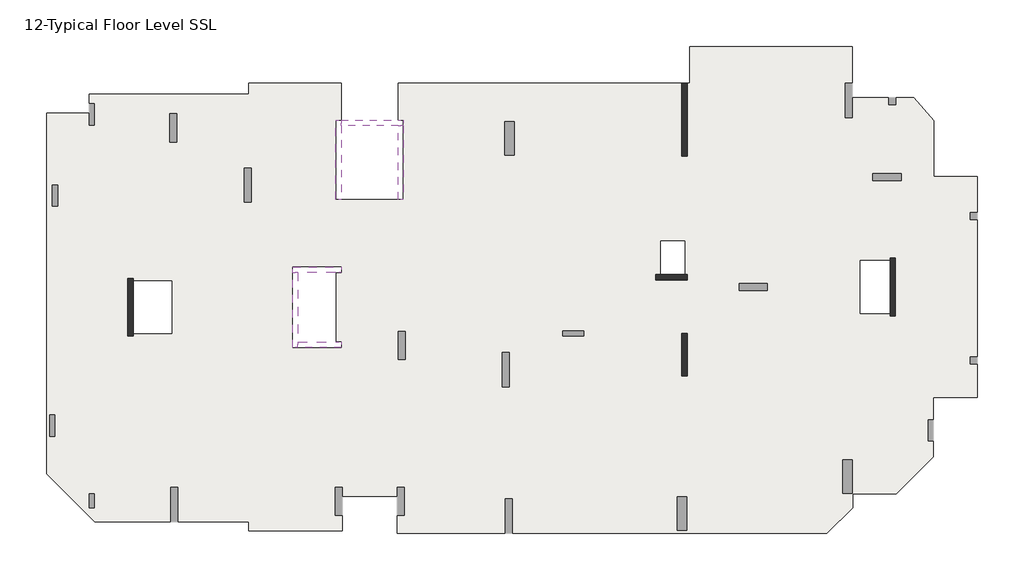
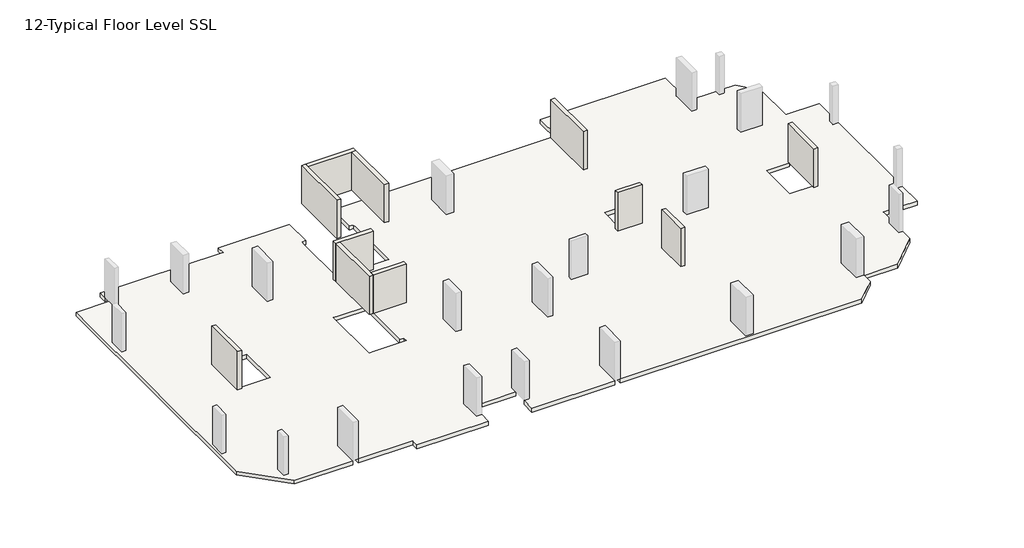
# One storey, part 1 of 2: 11 walls, 1 slab.
"""IFC4 building model written with IfcOpenShell, lengths in millimetres."""

from ifc_helpers import new_model, si_unit, origin, place, context, project, spatial, faceted_brep, element, save

model = new_model("IFC4")

# Units and contexts
model_context = context("Model", 3, world=origin())
ifc_project = project(units=[si_unit("LENGTHUNIT", "METRE", prefix="MILLI")], contexts=[model_context])

# Site, building, storey
site = spatial("IfcSite", under=ifc_project)
building = spatial("IfcBuilding", under=site)
storey = spatial("IfcBuildingStorey", under=building, Name="12-Typical Floor Level SSL", Elevation=30000.0)

# Slab
placement = place(None, origin())
element("IfcSlab", 1, ObjectType="Generic 300mm", at=placement, inside=storey, context=model_context, shape_type="Brep", body=[
    faceted_brep([(36192.0021644, 24072.000519, 29700.0), (36192.0021644, 26172.000519, 29700.0), (45446.0007483, 26172.000519, 29700.0), (45446.0007483, 24087.0, 29700.0), (45046.0007483, 24087.0, 29700.0), (45046.0007483, 22137.0, 29700.0), (45446.0007483, 22137.0, 29700.0), (45446.0007483, 23252.0000315, 29700.0), (47498.6337868, 23252.0000315, 29700.0), (47498.6337868, 22852.0, 29700.0), (47898.6337868, 22852.0, 29700.0), (47898.6337868, 23252.0000315, 29700.0), (48936.764334, 23252.0000315, 29700.0), (50076.0016214, 21956.8283806, 29700.0), (50076.0016214, 18780.0084406, 29700.0), (52549.9999998, 18780.0084406, 29700.0), (52549.9999998, 16712.0, 29700.0), (52149.9999998, 16712.0, 29700.0), (52149.9999998, 16312.0, 29700.0), (52549.9999998, 16312.0, 29700.0), (52549.9999998, 8504.0039609, 29700.0), (52149.9999998, 8504.0039609, 29700.0), (52149.9999998, 8104.0039609, 29700.0), (52549.9999998, 8104.0039609, 29700.0), (52549.9999998, 6204.0084406, 29700.0), (50046.0009271, 6204.0084406, 29700.0), (50046.0009271, 4931.9999929, 29700.0), (49746.0009271, 4931.9999929, 29700.0), (49746.0009271, 3731.9999929, 29700.0), (50046.0009271, 3731.9999929, 29700.0), (50046.0009271, 2810.5958657, 29700.0), (47943.4055804, 708.000519, 29700.0), (45456.0017287, 708.000519, 29700.0), (45456.0017287, -61.7051085, 29700.0), (43990.7023722, -1527.004465, 29700.0), (26113.9999998, -1527.004465, 29700.0), (26113.9999998, 422.995535, 29700.0), (25713.9999998, 422.995535, 29700.0), (25713.9999998, -1527.004465, 29700.0), (19569.9997488, -1527.004465, 29700.0), (19569.9997488, -512.0044652, 29700.0), (19969.9997488, -512.0044652, 29700.0), (19969.9997488, 1087.9955348, 29700.0), (19569.9997488, 1087.9955348, 29700.0), (19569.9997488, 564.000519, 29700.0), (16429.9999981, 564.000519, 29700.0), (16429.9999981, 1088.0, 29700.0), (16029.9999981, 1088.0, 29700.0), (16029.9999981, -512.0, 29700.0), (16429.9999981, -512.0, 29700.0), (16429.9999981, -1391.999481, 29700.0), (11136.0000923, -1391.999481, 29700.0), (11136.0000923, -866.9999847, 29700.0), (7082.0000416, -866.9999847, 29700.0), (7082.0000416, 1083.0000153, 29700.0), (6682.0000416, 1083.0000153, 29700.0), (6682.0000416, -866.9999847, 29700.0), (2364.4419097, -866.9999847, 29700.0), (-372.0, 1869.441925, 29700.0), (-372.0, 22380.0004589, 29700.0), (2052.0, 22380.0004589, 29700.0), (2052.0, 21708.0000656, 29700.0), (2352.0, 21708.0000656, 29700.0), (2352.0, 22908.0000656, 29700.0), (2052.0, 22908.0000656, 29700.0), (2052.0, 23472.000519, 29700.0), (11136.0000923, 23472.000519, 29700.0), (11136.0000923, 24072.000519, 29700.0), (16380.0000168, 24072.000519, 29700.0), (16380.0000168, 21972.0, 29700.0), (16079.9999997, 21972.0, 29700.0), (16079.9999997, 21672.0, 29700.0), (16079.9999997, 17468.0, 29700.0), (16379.9999997, 17468.0, 29700.0), (19619.9999997, 17468.0, 29700.0), (19919.9999997, 17468.0, 29700.0), (19919.9999997, 21672.0, 29700.0), (19919.9999997, 21972.0, 29700.0), (19619.9997365, 21972.0, 29700.0), (19619.9997365, 24072.000519, 29700.0), (35747.9999998, 24072.000519, 29700.0), (35747.9999998, 19932.0, 29700.0), (36047.9999998, 19932.0, 29700.0), (36047.9999998, 24072.000519, 29700.0), (16079.9999907, 9359.999998, 29700.0), (16079.9999907, 13320.0000002, 29700.0), (16380.0000168, 13320.0000002, 29700.0), (16380.0000168, 13620.0000002, 29700.0), (13919.9999907, 13620.0000002, 29700.0), (13619.9999907, 13620.0000002, 29700.0), (13619.9999907, 13320.0000002, 29700.0), (13619.9999907, 9359.999998, 29700.0), (13619.9999907, 9059.999998, 29700.0), (13919.9999907, 9059.999998, 29700.0), (16380.0000168, 9059.999998, 29700.0), (16380.0000168, 9359.999998, 29700.0), (4548.0000034, 9840.0000003, 29700.0), (6743.9999995, 9840.0000003, 29700.0), (6743.9999995, 12840.0000003, 29700.0), (4548.0000034, 12840.0000003, 29700.0), (4548.0000025, 12984.0000001, 29700.0), (4248.0000025, 12984.0000001, 29700.0), (4248.0000025, 9696.0, 29700.0), (4548.0000025, 9696.0, 29700.0), (47580.0014798, 13992.0079177, 29700.0), (45900.001729, 13992.0079177, 29700.0), (45900.001729, 10992.0079181, 29700.0), (47580.0014798, 10992.0079181, 29700.0), (47580.0014811, 10848.0079202, 29700.0), (47880.0014811, 10848.0079202, 29700.0), (47880.0014811, 14136.0000002, 29700.0), (47580.0014811, 14136.0000002, 29700.0), (35904.002157, 15108.0000083, 29700.0), (34548.0015145, 15108.0000083, 29700.0), (34548.0015145, 13199.9999992, 29700.0), (34248.0015201, 13199.9999992, 29700.0), (34248.0015201, 12899.9999992, 29700.0), (36048.0015201, 12899.9999992, 29700.0), (36048.0015201, 13199.9999992, 29700.0), (35904.002157, 13199.9999992, 29700.0), (257.9999999, 17088.0, 29700.0), (257.9999999, 18288.0, 29700.0), (-42.0000001, 18288.0, 29700.0), (-42.0000001, 17088.0, 29700.0), (108.001803, 4001.9999858, 29700.0), (108.001803, 5201.9999858, 29700.0), (-191.998197, 5201.9999858, 29700.0), (-191.998197, 4001.9999858, 29700.0), (30175.9999998, 9996.0000019, 29700.0), (28975.9999998, 9996.0000019, 29700.0), (28975.9999998, 9696.0000019, 29700.0), (30175.9999998, 9696.0000019, 29700.0), (7021.9999999, 20740.0000078, 29700.0), (7021.9999999, 22340.0000078, 29700.0), (6621.9999999, 22340.0000078, 29700.0), (6621.9999999, 20740.0000078, 29700.0), (48205.9993605, 18950.0, 29700.0), (46605.9993605, 18950.0, 29700.0), (46605.9993605, 18550.0, 29700.0), (48205.9993605, 18550.0, 29700.0), (20030.000009, 8355.9999979, 29700.0), (20030.000009, 9955.9999979, 29700.0), (19630.000009, 9955.9999979, 29700.0), (19630.000009, 8355.9999979, 29700.0), (11270.0000427, 17312.9999996, 29700.0), (11270.0000427, 19262.9999996, 29700.0), (10870.0000427, 19262.9999996, 29700.0), (10870.0000427, 17312.9999996, 29700.0), (40598.0014887, 12692.0079212, 29700.0), (38998.0014887, 12692.0079212, 29700.0), (38998.0014887, 12292.0079212, 29700.0), (40598.0014887, 12292.0079212, 29700.0), (2352.0, -72.0, 29700.0), (2352.0, 728.0, 29700.0), (2052.0, 728.0, 29700.0), (2052.0, -72.0, 29700.0), (25934.0000455, 6801.0001824, 29700.0), (25934.0000455, 8751.0001824, 29700.0), (25534.0000455, 8751.0001824, 29700.0), (25534.0000455, 6801.0001824, 29700.0), (36035.9999998, -1351.9992017, 29700.0), (36035.9999998, 548.0007983, 29700.0), (35485.9999998, 548.0007983, 29700.0), (35485.9999998, -1351.9992017, 29700.0), (45443.9999998, 748.0, 29700.0), (45443.9999998, 2648.0, 29700.0), (44893.9999998, 2648.0, 29700.0), (44893.9999998, 748.0, 29700.0), (26218.9999998, 20000.0, 29700.0), (26218.9999998, 21900.0, 29700.0), (25668.9999998, 21900.0, 29700.0), (25668.9999998, 20000.0, 29700.0), (35748.0054035, 9840.0000002, 29700.0), (35748.0054035, 7428.0000762, 29700.0), (36048.0054035, 7428.0000762, 29700.0), (36048.0054035, 9840.0000002, 29700.0), (36192.0021644, 26172.000519, 30000.0), (36192.0021644, 24072.000519, 30000.0), (36047.9999998, 24072.000519, 30000.0), (36047.9999998, 19932.0, 30000.0), (35747.9999998, 19932.0, 30000.0), (35747.9999998, 24072.000519, 30000.0), (19619.9997365, 24072.000519, 30000.0), (19619.9997365, 21972.0, 30000.0), (19919.9999997, 21972.0, 30000.0), (19919.9999997, 21672.0, 30000.0), (19919.9999997, 17468.0, 30000.0), (19619.9999997, 17468.0, 30000.0), (16379.9999997, 17468.0, 30000.0), (16079.9999997, 17468.0, 30000.0), (16079.9999997, 21672.0, 30000.0), (16079.9999997, 21972.0, 30000.0), (16380.0000168, 21972.0, 30000.0), (16380.0000168, 24072.000519, 30000.0), (11136.0000923, 24072.000519, 30000.0), (11136.0000923, 23472.000519, 30000.0), (2052.0, 23472.000519, 30000.0), (2052.0, 22908.0000656, 30000.0), (2352.0, 22908.0000656, 30000.0), (2352.0, 21708.0000656, 30000.0), (2052.0, 21708.0000656, 30000.0), (2052.0, 22380.0004589, 30000.0), (-372.0, 22380.0004589, 30000.0), (-372.0, 1869.441925, 30000.0), (2364.4419097, -866.9999847, 30000.0), (6682.0000416, -866.9999847, 30000.0), (6682.0000416, 1083.0000153, 30000.0), (7082.0000416, 1083.0000153, 30000.0), (7082.0000416, -866.9999847, 30000.0), (11136.0000923, -866.9999847, 30000.0), (11136.0000923, -1391.999481, 30000.0), (16429.9999981, -1391.999481, 30000.0), (16429.9999981, -512.0, 30000.0), (16029.9999981, -512.0, 30000.0), (16029.9999981, 1088.0, 30000.0), (16429.9999981, 1088.0, 30000.0), (16429.9999981, 564.000519, 30000.0), (19569.9997488, 564.000519, 30000.0), (19569.9997488, 1087.9955348, 30000.0), (19969.9997488, 1087.9955348, 30000.0), (19969.9997488, -512.0044652, 30000.0), (19569.9997488, -512.0044652, 30000.0), (19569.9997488, -1527.004465, 30000.0), (25713.9999998, -1527.004465, 30000.0), (25713.9999998, 422.995535, 30000.0), (26113.9999998, 422.995535, 30000.0), (26113.9999998, -1527.004465, 30000.0), (43990.7023722, -1527.004465, 30000.0), (45456.0017287, -61.7051085, 30000.0), (45456.0017287, 708.000519, 30000.0), (47943.4055804, 708.000519, 30000.0), (50046.0009271, 2810.5958657, 30000.0), (50046.0009271, 3731.9999929, 30000.0), (49746.0009271, 3731.9999929, 30000.0), (49746.0009271, 4931.9999929, 30000.0), (50046.0009271, 4931.9999929, 30000.0), (50046.0009271, 6204.0084406, 30000.0), (52549.9999998, 6204.0084406, 30000.0), (52549.9999998, 8104.0039609, 30000.0), (52149.9999998, 8104.0039609, 30000.0), (52149.9999998, 8504.0039609, 30000.0), (52549.9999998, 8504.0039609, 30000.0), (52549.9999998, 16312.0, 30000.0), (52149.9999998, 16312.0, 30000.0), (52149.9999998, 16712.0, 30000.0), (52549.9999998, 16712.0, 30000.0), (52549.9999998, 18780.0084406, 30000.0), (50076.0016214, 18780.0084406, 30000.0), (50076.0016214, 21956.8283806, 30000.0), (48936.764334, 23252.0000315, 30000.0), (47898.6337868, 23252.0000315, 30000.0), (47898.6337868, 22852.0, 30000.0), (47498.6337868, 22852.0, 30000.0), (47498.6337868, 23252.0000315, 30000.0), (45446.0006898, 23252.0000315, 30000.0), (45446.0007483, 22137.0, 30000.0), (45046.0007483, 22137.0, 30000.0), (45046.0007483, 24087.0, 30000.0), (45446.0007483, 24087.0, 30000.0), (45446.0007483, 26172.000519, 30000.0), (16079.9999907, 13320.0000002, 30000.0), (16079.9999907, 9359.999998, 30000.0), (16380.0000168, 9359.999998, 30000.0), (16380.0000168, 9059.999998, 30000.0), (13919.9999907, 9059.999998, 30000.0), (13619.9999907, 9059.999998, 30000.0), (13619.9999907, 9359.999998, 30000.0), (13619.9999907, 13320.0000002, 30000.0), (13619.9999907, 13620.0000002, 30000.0), (13919.9999907, 13620.0000002, 30000.0), (16380.0000168, 13620.0000002, 30000.0), (16380.0000168, 13320.0000002, 30000.0), (6743.9999995, 9840.0000003, 30000.0), (4548.0000034, 9840.0000003, 30000.0), (4548.0000025, 9696.0, 30000.0), (4248.0000025, 9696.0, 30000.0), (4248.0000025, 12984.0000001, 30000.0), (4548.0000025, 12984.0000001, 30000.0), (4548.0000025, 12840.0000003, 30000.0), (6743.9999995, 12840.0000003, 30000.0), (45900.001729, 13992.0079177, 30000.0), (47580.0014798, 13992.0079177, 30000.0), (47580.0014811, 14136.0000002, 30000.0), (47880.0014811, 14136.0000002, 30000.0), (47880.0014811, 10848.0079202, 30000.0), (47580.0014811, 10848.0079202, 30000.0), (47580.0014811, 10992.0079181, 30000.0), (45900.001729, 10992.0079181, 30000.0), (34548.0015145, 15108.0000083, 30000.0), (35904.002157, 15108.0000083, 30000.0), (35904.002157, 13199.9999992, 30000.0), (36048.0015201, 13199.9999992, 30000.0), (36048.0015201, 12899.9999992, 30000.0), (34248.0015201, 12899.9999992, 30000.0), (34248.0015201, 13199.9999992, 30000.0), (34548.0015145, 13199.9999992, 30000.0), (257.9999999, 18288.0, 30000.0), (257.9999999, 17088.0, 30000.0), (-42.0000001, 17088.0, 30000.0), (-42.0000001, 18288.0, 30000.0), (108.001803, 5201.9999858, 30000.0), (108.001803, 4001.9999858, 30000.0), (-191.998197, 4001.9999858, 30000.0), (-191.998197, 5201.9999858, 30000.0), (28975.9999998, 9996.0000019, 30000.0), (30175.9999998, 9996.0000019, 30000.0), (30175.9999998, 9696.0000019, 30000.0), (28975.9999998, 9696.0000019, 30000.0), (7021.9999999, 22340.0000078, 30000.0), (7021.9999999, 20740.0000078, 30000.0), (6621.9999999, 20740.0000078, 30000.0), (6621.9999999, 22340.0000078, 30000.0), (46605.9993605, 18950.0, 30000.0), (48205.9993605, 18950.0, 30000.0), (48205.9993605, 18550.0, 30000.0), (46605.9993605, 18550.0, 30000.0), (20030.000009, 9955.9999979, 30000.0), (20030.000009, 8355.9999979, 30000.0), (19630.000009, 8355.9999979, 30000.0), (19630.000009, 9955.9999979, 30000.0), (11270.0000427, 19262.9999996, 30000.0), (11270.0000427, 17312.9999996, 30000.0), (10870.0000427, 17312.9999996, 30000.0), (10870.0000427, 19262.9999996, 30000.0), (38998.0014887, 12692.0079212, 30000.0), (40598.0014887, 12692.0079212, 30000.0), (40598.0014887, 12292.0079212, 30000.0), (38998.0014887, 12292.0079212, 30000.0), (2352.0, 728.0, 30000.0), (2352.0, -72.0, 30000.0), (2052.0, -72.0, 30000.0), (2052.0, 728.0, 30000.0), (25934.0000455, 8751.0001824, 30000.0), (25934.0000455, 6801.0001824, 30000.0), (25534.0000455, 6801.0001824, 30000.0), (25534.0000455, 8751.0001824, 30000.0), (36035.9999998, 548.0007983, 30000.0), (36035.9999998, -1351.9992017, 30000.0), (35485.9999998, -1351.9992017, 30000.0), (35485.9999998, 548.0007983, 30000.0), (45443.9999998, 2648.0, 30000.0), (45443.9999998, 748.0, 30000.0), (44893.9999998, 748.0, 30000.0), (44893.9999998, 2648.0, 30000.0), (26218.9999998, 21900.0, 30000.0), (26218.9999998, 20000.0, 30000.0), (25668.9999998, 20000.0, 30000.0), (25668.9999998, 21900.0, 30000.0), (35748.0054035, 7428.0000762, 30000.0), (35748.0054035, 9840.0000002, 30000.0), (36048.0054035, 9840.0000002, 30000.0), (36048.0054035, 7428.0000762, 30000.0)], [[[0, 1, 2, 3, 4, 5, 6, 7, 8, 9, 10, 11, 12, 13, 14, 15, 16, 17, 18, 19, 20, 21, 22, 23, 24, 25, 26, 27, 28, 29, 30, 31, 32, 33, 34, 35, 36, 37, 38, 39, 40, 41, 42, 43, 44, 45, 46, 47, 48, 49, 50, 51, 52, 53, 54, 55, 56, 57, 58, 59, 60, 61, 62, 63, 64, 65, 66, 67, 68, 69, 70, 71, 72, 73, 74, 75, 76, 77, 78, 79, 80, 81, 82, 83], [84, 85, 86, 87, 88, 89, 90, 91, 92, 93, 94, 95], [96, 97, 98, 99, 100, 101, 102, 103], [104, 105, 106, 107, 108, 109, 110, 111], [112, 113, 114, 115, 116, 117, 118, 119], [120, 121, 122, 123], [124, 125, 126, 127], [128, 129, 130, 131], [132, 133, 134, 135], [136, 137, 138, 139], [140, 141, 142, 143], [144, 145, 146, 147], [148, 149, 150, 151], [152, 153, 154, 155], [156, 157, 158, 159], [160, 161, 162, 163], [164, 165, 166, 167], [168, 169, 170, 171], [172, 173, 174, 175]], [[176, 177, 178, 179, 180, 181, 182, 183, 184, 185, 186, 187, 188, 189, 190, 191, 192, 193, 194, 195, 196, 197, 198, 199, 200, 201, 202, 203, 204, 205, 206, 207, 208, 209, 210, 211, 212, 213, 214, 215, 216, 217, 218, 219, 220, 221, 222, 223, 224, 225, 226, 227, 228, 229, 230, 231, 232, 233, 234, 235, 236, 237, 238, 239, 240, 241, 242, 243, 244, 245, 246, 247, 248, 249, 250, 251, 252, 253, 254, 255, 256, 257, 258, 259], [260, 261, 262, 263, 264, 265, 266, 267, 268, 269, 270, 271], [272, 273, 274, 275, 276, 277, 278, 279], [280, 281, 282, 283, 284, 285, 286, 287], [288, 289, 290, 291, 292, 293, 294, 295], [296, 297, 298, 299], [300, 301, 302, 303], [304, 305, 306, 307], [308, 309, 310, 311], [312, 313, 314, 315], [316, 317, 318, 319], [320, 321, 322, 323], [324, 325, 326, 327], [328, 329, 330, 331], [332, 333, 334, 335], [336, 337, 338, 339], [340, 341, 342, 343], [344, 345, 346, 347], [348, 349, 350, 351]], [[68, 193, 192, 69]], [[182, 79, 78, 183]], [[79, 182, 181, 80]], [[177, 0, 83, 178]], [[1, 0, 177, 176]], [[2, 1, 176, 259]], [[3, 2, 259, 258]], [[249, 12, 11, 250]], [[7, 254, 253, 8]], [[13, 12, 249, 248]], [[14, 13, 248, 247]], [[15, 14, 247, 246]], [[15, 246, 245, 16]], [[237, 24, 23, 238]], [[19, 242, 241, 20]], [[25, 24, 237, 236]], [[25, 236, 235, 26]], [[231, 30, 29, 232]], [[32, 31, 230, 229]], [[33, 32, 229, 228]], [[34, 33, 228, 227]], [[34, 227, 226, 35]], [[222, 39, 38, 223]], [[39, 222, 221, 40]], [[45, 44, 217, 216]], [[211, 50, 49, 212]], [[51, 50, 211, 210]], [[52, 51, 210, 209]], [[52, 209, 208, 53]], [[204, 57, 56, 205]], [[58, 57, 204, 203]], [[59, 58, 203, 202]], [[60, 59, 202, 201]], [[196, 65, 64, 197]], [[66, 65, 196, 195]], [[67, 66, 195, 194]], [[68, 67, 194, 193]], [[31, 30, 231, 230]], [[85, 84, 261, 260]], [[72, 189, 188, 187, 186, 75, 74, 73]], [[272, 97, 96, 273]], [[97, 272, 279, 98]], [[98, 279, 278, 99]], [[280, 105, 104, 281]], [[105, 280, 287, 106]], [[106, 287, 286, 107]], [[112, 289, 288, 113]], [[113, 288, 295, 114]], [[289, 112, 119, 290]], [[62, 199, 198, 63]], [[199, 62, 61, 200]], [[200, 61, 60, 201]], [[63, 198, 197, 64]], [[120, 297, 296, 121]], [[297, 120, 123, 298]], [[298, 123, 122, 299]], [[299, 122, 121, 296]], [[124, 301, 300, 125]], [[301, 124, 127, 302]], [[302, 127, 126, 303]], [[303, 126, 125, 300]], [[28, 233, 232, 29]], [[233, 28, 27, 234]], [[234, 27, 26, 235]], [[128, 305, 304, 129]], [[305, 128, 131, 306]], [[306, 131, 130, 307]], [[307, 130, 129, 304]], [[132, 309, 308, 133]], [[309, 132, 135, 310]], [[310, 135, 134, 311]], [[311, 134, 133, 308]], [[41, 220, 219, 42]], [[220, 41, 40, 221]], [[43, 218, 217, 44]], [[218, 43, 42, 219]], [[136, 313, 312, 137]], [[313, 136, 139, 314]], [[314, 139, 138, 315]], [[315, 138, 137, 312]], [[140, 317, 316, 141]], [[317, 140, 143, 318]], [[318, 143, 142, 319]], [[319, 142, 141, 316]], [[215, 46, 45, 216]], [[48, 213, 212, 49]], [[213, 48, 47, 214]], [[214, 47, 46, 215]], [[144, 321, 320, 145]], [[321, 144, 147, 322]], [[322, 147, 146, 323]], [[323, 146, 145, 320]], [[207, 54, 53, 208]], [[55, 206, 205, 56]], [[206, 55, 54, 207]], [[225, 36, 35, 226]], [[37, 224, 223, 38]], [[224, 37, 36, 225]], [[6, 255, 254, 7]], [[255, 6, 5, 256]], [[256, 5, 4, 257]], [[257, 4, 3, 258]], [[148, 325, 324, 149]], [[325, 148, 151, 326]], [[326, 151, 150, 327]], [[327, 150, 149, 324]], [[152, 329, 328, 153]], [[329, 152, 155, 330]], [[330, 155, 154, 331]], [[331, 154, 153, 328]], [[156, 333, 332, 157]], [[333, 156, 159, 334]], [[334, 159, 158, 335]], [[335, 158, 157, 332]], [[160, 337, 336, 161]], [[337, 160, 163, 338]], [[338, 163, 162, 339]], [[339, 162, 161, 336]], [[164, 341, 340, 165]], [[341, 164, 167, 342]], [[342, 167, 166, 343]], [[343, 166, 165, 340]], [[168, 345, 344, 169]], [[345, 168, 171, 346]], [[346, 171, 170, 347]], [[347, 170, 169, 344]], [[70, 191, 190, 189, 72, 71]], [[191, 70, 69, 192]], [[77, 184, 183, 78]], [[184, 77, 76, 75, 186, 185]], [[271, 86, 85, 260]], [[87, 270, 269, 268, 89, 88]], [[86, 271, 270, 87]], [[89, 268, 267, 266, 265, 92, 91, 90]], [[92, 265, 264, 263, 94, 93]], [[95, 262, 261, 84]], [[262, 95, 94, 263]], [[277, 100, 99, 278]], [[103, 274, 273, 96]], [[101, 276, 275, 102]], [[100, 277, 276, 101]], [[274, 103, 102, 275]], [[116, 293, 292, 117]], [[118, 291, 290, 119]], [[294, 115, 114, 295]], [[117, 292, 291, 118]], [[293, 116, 115, 294]], [[172, 349, 348, 173]], [[174, 351, 350, 175]], [[173, 348, 351, 174]], [[349, 172, 175, 350]], [[285, 108, 107, 286]], [[111, 282, 281, 104]], [[109, 284, 283, 110]], [[108, 285, 284, 109]], [[282, 111, 110, 283]], [[82, 179, 178, 83]], [[180, 81, 80, 181]], [[179, 82, 81, 180]], [[18, 243, 242, 19]], [[243, 18, 17, 244]], [[244, 17, 16, 245]], [[10, 251, 250, 11]], [[251, 10, 9, 252]], [[252, 9, 8, 253]], [[22, 239, 238, 23]], [[239, 22, 21, 240]], [[240, 21, 20, 241]]]),
])

# Walls
element("IfcWall", 2, ObjectType="Shear Walls 300mm", at=placement, inside=storey, context=model_context, shape_type="Brep", body=[
    faceted_brep([(4548.0000025, 9696.0, 30000.0), (4548.0000025, 12984.0000001, 30000.0), (4548.0000025, 12984.0000001, 32700.0), (4548.0000025, 12984.0000001, 33000.0), (4548.0000025, 12840.0000003, 33000.0), (4548.0000025, 9840.0000003, 33000.0), (4548.0000025, 9696.0, 33000.0), (4548.0000025, 9696.0, 32700.0), (4248.0000025, 9696.0, 30000.0), (4248.0000025, 9696.0, 32700.0), (4248.0000025, 9696.0, 33000.0), (4248.0000025, 12984.0000001, 33000.0), (4248.0000025, 12984.0000001, 32700.0), (4248.0000025, 12984.0000001, 30000.0)], [[[0, 1, 2, 3, 4, 5, 6, 7]], [[8, 9, 10, 11, 12, 13]], [[1, 0, 8, 13]], [[3, 2, 1, 13, 12, 11]], [[6, 5, 4, 3, 11, 10]], [[0, 7, 6, 10, 9, 8]]]),
])
element("IfcWall", 3, ObjectType="Shear Walls 300mm", at=placement, inside=storey, context=model_context, shape_type="Brep", body=[
    faceted_brep([(34248.0015201, 12899.9999992, 30000.0), (36048.0015201, 12899.9999992, 30000.0), (36048.0015201, 12899.9999992, 32700.0), (36048.0015201, 12899.9999992, 33000.0), (34248.0015201, 12899.9999992, 33000.0), (34248.0015201, 12899.9999992, 32700.0), (34248.0015201, 13199.9999992, 30000.0), (34248.0015201, 13199.9999992, 32700.0), (34248.0015201, 13199.9999992, 33000.0), (34548.0015145, 13199.9999992, 33000.0), (35904.002157, 13199.9999992, 33000.0), (36048.0015201, 13199.9999992, 33000.0), (36048.0015201, 13199.9999992, 32700.0), (36048.0015201, 13199.9999992, 30000.0)], [[[0, 1, 2, 3, 4, 5]], [[6, 7, 8, 9, 10, 11, 12, 13]], [[1, 0, 6, 13]], [[3, 2, 1, 13, 12, 11]], [[4, 3, 11, 10, 9, 8]], [[0, 5, 4, 8, 7, 6]]]),
])
element("IfcWall", 4, ObjectType="Shear Walls 300mm", at=placement, inside=storey, context=model_context, shape_type="Brep", body=[
    faceted_brep([(35748.0054035, 9840.0000002, 30000.0), (35748.0054035, 7428.0000762, 30000.0), (35748.0054035, 7428.0000762, 32700.0), (35748.0054035, 7428.0000762, 33000.0), (35748.0054035, 9840.0000002, 33000.0), (35748.0054035, 9840.0000002, 32700.0), (36048.0054035, 9840.0000002, 30000.0), (36048.0054035, 9840.0000002, 32700.0), (36048.0054035, 9840.0000002, 33000.0), (36048.0054035, 7428.0000762, 33000.0), (36048.0054035, 7428.0000762, 32700.0), (36048.0054035, 7428.0000762, 30000.0)], [[[0, 1, 2, 3, 4, 5]], [[6, 7, 8, 9, 10, 11]], [[1, 0, 6, 11]], [[3, 2, 1, 11, 10, 9]], [[4, 3, 9, 8]], [[0, 5, 4, 8, 7, 6]]]),
])
element("IfcWall", 5, ObjectType="Shear Walls 300mm", at=placement, inside=storey, context=model_context, shape_type="Brep", body=[
    faceted_brep([(47580.0014811, 14136.0000002, 30000.0), (47580.0014811, 10848.0079202, 30000.0), (47580.0014811, 10848.0079202, 32700.0), (47580.0014811, 10848.0079202, 33000.0), (47580.0014811, 10992.0079181, 33000.0), (47580.0014811, 13992.0079177, 33000.0), (47580.0014811, 14136.0000002, 33000.0), (47580.0014811, 14136.0000002, 32700.0), (47880.0014811, 14136.0000002, 30000.0), (47880.0014811, 14136.0000002, 32700.0), (47880.0014811, 14136.0000002, 33000.0), (47880.0014811, 10848.0079202, 33000.0), (47880.0014811, 10848.0079202, 32700.0), (47880.0014811, 10848.0079202, 30000.0)], [[[0, 1, 2, 3, 4, 5, 6, 7]], [[8, 9, 10, 11, 12, 13]], [[1, 0, 8, 13]], [[3, 2, 1, 13, 12, 11]], [[6, 5, 4, 3, 11, 10]], [[0, 7, 6, 10, 9, 8]]]),
])
element("IfcWall", 6, ObjectType="Shear Walls 300mm", at=placement, inside=storey, context=model_context, shape_type="Brep", body=[
    faceted_brep([(36047.9999998, 19932.0, 30000.0), (36047.9999998, 24072.0078999, 30000.0), (36047.9999998, 24072.0078999, 33000.0), (36047.9999998, 19932.0, 33000.0), (36047.9999998, 19932.0, 32700.0), (35747.9999998, 19932.0, 30000.0), (35747.9999998, 19932.0, 32700.0), (35747.9999998, 19932.0, 33000.0), (35747.9999998, 24072.0078999, 33000.0), (35747.9999998, 24072.0078999, 30000.0)], [[[0, 1, 2, 3, 4]], [[5, 6, 7, 8, 9]], [[1, 0, 5, 9]], [[2, 1, 9, 8]], [[3, 2, 8, 7]], [[0, 4, 3, 7, 6, 5]]]),
])
element("IfcWall", 7, ObjectType="Shear Walls 300mm", at=placement, inside=storey, context=model_context, shape_type="Brep", body=[
    faceted_brep([(16379.9999997, 21972.0, 36000.0), (16379.9999997, 21672.0, 36000.0), (16379.9999997, 17468.0, 36000.0), (16379.9999997, 17468.0, 33000.0), (16379.9999997, 21672.0, 33000.0), (16379.9999997, 21972.0, 33000.0), (16079.9999997, 17468.0, 36000.0), (16079.9999997, 21972.0, 36000.0), (16079.9999997, 21972.0, 35700.0), (16079.9999997, 21972.0, 33000.0), (16079.9999997, 17468.0, 33000.0), (16079.9999997, 17468.0, 35700.0)], [[[0, 1, 2, 3, 4, 5]], [[6, 7, 8, 9, 10, 11]], [[2, 1, 0, 7, 6]], [[2, 6, 11, 10, 3]], [[3, 10, 9, 5, 4]], [[0, 5, 9, 8, 7]]]),
])
element("IfcWall", 8, ObjectType="Shear Walls 300mm", at=placement, inside=storey, context=model_context, shape_type="Brep", body=[
    faceted_brep([(16379.9999997, 21972.0, 36000.0), (19619.9997365, 21972.0, 36000.0), (19919.9999997, 21972.0, 36000.0), (19919.9999997, 21972.0, 35700.0), (19919.9999997, 21972.0, 33000.0), (16379.9999997, 21972.0, 33000.0), (19919.9999997, 21672.0, 36000.0), (19619.9999997, 21672.0, 36000.0), (16379.9999997, 21672.0, 36000.0), (16379.9999997, 21672.0, 33000.0), (19619.9999997, 21672.0, 33000.0), (19919.9999997, 21672.0, 33000.0)], [[[0, 1, 2, 3, 4, 5]], [[6, 7, 8, 9, 10, 11]], [[2, 1, 0, 8, 7, 6]], [[8, 0, 5, 9]], [[9, 5, 4, 11, 10]], [[4, 3, 2, 6, 11]]]),
])
element("IfcWall", 9, ObjectType="Shear Walls 300mm", at=placement, inside=storey, context=model_context, shape_type="Brep", body=[
    faceted_brep([(19919.9999997, 21672.0, 36000.0), (19919.9999997, 17468.0, 36000.0), (19919.9999997, 17468.0, 35700.0), (19919.9999997, 17468.0, 33000.0), (19919.9999997, 21672.0, 33000.0), (19619.9999997, 17468.0, 36000.0), (19619.9999997, 21672.0, 36000.0), (19619.9999997, 21672.0, 33000.0), (19619.9999997, 17468.0, 33000.0)], [[[0, 1, 2, 3, 4]], [[5, 6, 7, 8]], [[1, 0, 6, 5]], [[1, 5, 8, 3, 2]], [[6, 0, 4, 7]], [[4, 3, 8, 7]]]),
])
element("IfcWall", 10, ObjectType="Shear Walls 300mm", at=placement, inside=storey, context=model_context, shape_type="Brep", body=[
    faceted_brep([(16380.0000168, 13320.0000002, 36000.0), (16079.9999907, 13320.0000002, 36000.0), (13919.9999907, 13320.0000002, 36000.0), (13619.9999907, 13320.0000002, 36000.0), (13619.9999907, 13320.0000002, 33000.0), (13919.9999907, 13320.0000002, 33000.0), (16380.0000168, 13320.0000002, 33000.0), (16380.0000168, 13320.0000002, 35700.0), (13619.9999907, 13620.0000002, 36000.0), (16380.0000168, 13620.0000002, 36000.0), (16380.0000168, 13620.0000002, 35700.0), (16380.0000168, 13620.0000002, 33000.0), (13619.9999907, 13620.0000002, 33000.0), (13619.9999907, 13620.0000002, 35700.0)], [[[0, 1, 2, 3, 4, 5, 6, 7]], [[8, 9, 10, 11, 12, 13]], [[9, 0, 7, 6, 11, 10]], [[3, 2, 1, 0, 9, 8]], [[11, 6, 5, 4, 12]], [[4, 3, 8, 13, 12]]]),
])
element("IfcWall", 11, ObjectType="Shear Walls 300mm", at=placement, inside=storey, context=model_context, shape_type="Brep", body=[
    faceted_brep([(13919.9999907, 13320.0000002, 36000.0), (13919.9999907, 9359.999998, 36000.0), (13919.9999907, 9059.999998, 36000.0), (13919.9999907, 9059.999998, 33000.0), (13919.9999907, 9359.999998, 33000.0), (13919.9999907, 13320.0000002, 33000.0), (13619.9999907, 9059.999998, 36000.0), (13619.9999907, 13320.0000002, 36000.0), (13619.9999907, 13320.0000002, 33000.0), (13619.9999907, 9059.999998, 33000.0), (13619.9999907, 9059.999998, 35700.0)], [[[0, 1, 2, 3, 4, 5]], [[6, 7, 8, 9, 10]], [[2, 1, 0, 7, 6]], [[7, 0, 5, 8]], [[8, 5, 4, 3, 9]], [[3, 2, 6, 10, 9]]]),
])
element("IfcWall", 12, ObjectType="Shear Walls 300mm", at=placement, inside=storey, context=model_context, shape_type="Brep", body=[
    faceted_brep([(13919.9999907, 9359.999998, 36000.0), (16079.9999907, 9359.999998, 36000.0), (16380.0000168, 9359.999998, 36000.0), (16380.0000168, 9359.999998, 35700.0), (16380.0000168, 9359.999998, 33000.0), (13919.9999907, 9359.999998, 33000.0), (16380.0000168, 9059.999998, 36000.0), (13919.9999907, 9059.999998, 36000.0), (13919.9999907, 9059.999998, 33000.0), (16380.0000168, 9059.999998, 33000.0), (16380.0000168, 9059.999998, 35700.0)], [[[0, 1, 2, 3, 4, 5]], [[6, 7, 8, 9, 10]], [[2, 1, 0, 7, 6]], [[2, 6, 10, 9, 4, 3]], [[7, 0, 5, 8]], [[5, 4, 9, 8]]]),
])

save(model, "model.ifc")

# Revit data of these elements
# Type "Generic 300mm"
#   Function = 0
#   Layers, outside or top first: 300 mm "Concrete-RC" (function 1)
# Type "Shear Walls 300mm"
#   Layers, outside or top first: 300 mm "Concrete-RC" (function 1)
# Element 1 (IfcSlab, "Generic 300mm")
#   Height Offset From Level = 0 mm
#   built-in parameter 1001954 = 1
#   Phase Created = New Construction
#   Materials on its faces: "Concrete-RC"
# Elements 2, 3, 4, 5, 6 (IfcWall, "Shear Walls 300mm")
#   Top Offset = 0 mm
#   Base Offset = 0 mm
#   wall height = 3000 mm
#   Phase Created = New Construction
#   Base Constraint = 12-Typical Floor Level SSL
#   Top Constraint = 13-Typical Floor Level SSL
#   Materials on its faces: "Concrete-RC"
# Elements 7, 8, 9, 10, 11, 12 (IfcWall, "Shear Walls 300mm")
#   Top Offset = 0 mm
#   Base Offset = 0 mm
#   wall height = 6000 mm
#   Phase Created = New Construction
#   Base Constraint = 12-Typical Floor Level SSL
#   Top Constraint = 14-Roof Level SSL
#   Materials on its faces: "Concrete-RC"
# Materials
#   "Concrete-RC": class "Concrete", colour RGB 128 128 128, transparency 0, Description = "High strength concrete", Cost = 0
